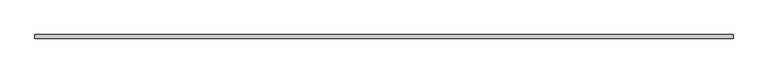
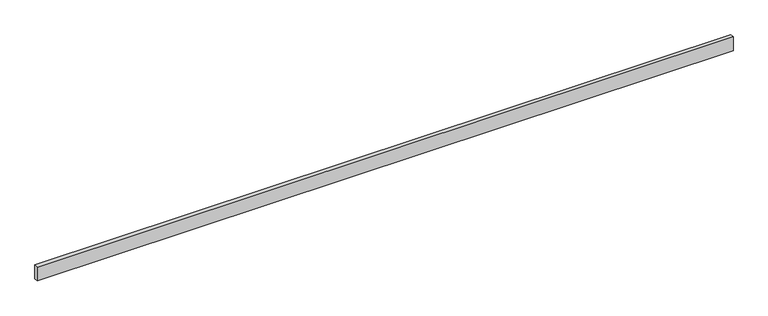
"""IFC4 building model written with IfcOpenShell, lengths in millimetres: proxy geometry, Generic Models 7:Generic Models 1:337419:Generic Models 1:337419 : Generic Models 7:Generic Models 1:337419:19 : Generic Models 7:Generic Models 1:337419:Generic Models 1:337419 : Generic Models 7:Generic Models 1:337419:301336."""

import ifcopenshell
import ifcopenshell.guid

model = None  # the IFC model being written
_history = None  # IfcOwnerHistory: only IFC2X3 demands one
_inside = {}  # id of a spatial element -> (the spatial element, [elements in it])
_under = {}  # id of a project, library or spatial element -> (it, [spatial elements below it])
_declared = {}  # id of a project -> (the project, [libraries it declares])
_typed = {}  # id of a type object -> (the type object, [elements of that type])
_made_of = {}  # id of a material, layer set ... -> (it, [elements and type objects made of it])


def new_model(schema):
    """Start an empty IFC model of exactly this schema.

    Asked for "IFC4X3", IfcOpenShell would pick the latest addendum, in which some entities
    have other attributes; the version numbers below select the first issue.
    IFC2X3 requires an IfcOwnerHistory on every rooted entity: one is made here for all.
    """
    global model, _history
    if schema == "IFC4X3":
        model = ifcopenshell.file(schema_version=(4, 3, 0, 0))
    else:
        model = ifcopenshell.file(schema=schema)
    _inside.clear()
    _under.clear()
    _declared.clear()
    _typed.clear()
    _made_of.clear()
    _history = None
    if model.schema == "IFC2X3":
        org = make("IfcOrganization", Name="unknown")
        user = make(
            "IfcPersonAndOrganization",
            ThePerson=make("IfcPerson", FamilyName="unknown"),
            TheOrganization=org,
        )
        app = make(
            "IfcApplication",
            ApplicationDeveloper=org,
            Version="unknown",
            ApplicationFullName="unknown",
            ApplicationIdentifier="unknown",
        )
        _history = make(
            "IfcOwnerHistory",
            OwningUser=user,
            OwningApplication=app,
            ChangeAction="ADDED",
            CreationDate=0,
        )
    return model


def make(cls, **values):
    """One entity of the class cls with the attributes given. An attribute that is None is left unset."""
    return model.create_entity(
        cls, **{name: value for name, value in values.items() if value is not None}
    )


def rooted(cls, **values):
    """An entity with a GlobalId (a new one), such as an element, a storey or a relation."""
    return make(cls, GlobalId=ifcopenshell.guid.new(), OwnerHistory=_history, **values)


def si_unit(unit_type, name, prefix=None):
    """IfcSIUnit, for example si_unit("LENGTHUNIT", "METRE", prefix="MILLI")."""
    return make("IfcSIUnit", UnitType=unit_type, Prefix=prefix, Name=name)


def assignment(units):
    """IfcUnitAssignment: the units of a project."""
    return None if units is None else make("IfcUnitAssignment", Units=units)


def point(xyz):
    """IfcCartesianPoint."""
    return None if xyz is None else make("IfcCartesianPoint", Coordinates=xyz)


def direction(xyz):
    """IfcDirection."""
    return None if xyz is None else make("IfcDirection", DirectionRatios=xyz)


def frame(location, z_axis=None, x_axis=None):
    """IfcAxis2Placement3D, a coordinate frame: its origin and axes. An axis left out is left unset."""
    return make(
        "IfcAxis2Placement3D",
        Location=point(location),
        Axis=direction(z_axis),
        RefDirection=direction(x_axis),
    )


def origin():
    """The frame at (0, 0, 0) with its axes left unset."""
    return frame((0.0, 0.0, 0.0))


def place(relative_to, where):
    """IfcLocalPlacement: puts the frame where relative to a parent placement (None: the world)."""
    return make(
        "IfcLocalPlacement", PlacementRelTo=relative_to, RelativePlacement=where
    )


def context(
    kind, dimensions, precision=None, world=None, true_north=None, identifier=None
):
    """IfcGeometricRepresentationContext, for example the 3D "Model" context."""
    return make(
        "IfcGeometricRepresentationContext",
        ContextIdentifier=identifier,
        ContextType=kind,
        CoordinateSpaceDimension=dimensions,
        Precision=precision,
        WorldCoordinateSystem=world,
        TrueNorth=true_north,
    )


def project(units=None, contexts=None):
    """IfcProject with its units and contexts."""
    return rooted(
        "IfcProject",
        Name="project",
        RepresentationContexts=contexts,
        UnitsInContext=assignment(units),
    )


def spatial(cls, under=None, at=None, **own):
    """A site, building, storey or space (cls), placed at a placement, below another one or the project."""
    s = rooted(cls, ObjectPlacement=at, **own)
    if under is not None:
        _under.setdefault(under.id(), (under, []))[1].append(s)
    return s


def polyline(points):
    """IfcPolyline through the points."""
    return make("IfcPolyline", Points=[point(p) for p in points])


def outline(outer, holes=None, kind="AREA"):
    """IfcArbitraryClosedProfileDef: a profile drawn as a closed curve; with holes, ...WithVoids."""
    if holes is None:
        return make("IfcArbitraryClosedProfileDef", ProfileType=kind, OuterCurve=outer)
    return make(
        "IfcArbitraryProfileDefWithVoids",
        ProfileType=kind,
        OuterCurve=outer,
        InnerCurves=holes,
    )


def extrude(swept, where, along, depth):
    """IfcExtrudedAreaSolid: the profile swept, set in the frame where, extruded along a direction by depth."""
    return make(
        "IfcExtrudedAreaSolid",
        SweptArea=swept,
        Position=where,
        ExtrudedDirection=direction(along),
        Depth=depth,
    )


def shape(context_of_items, identifier, shape_type, items):
    """IfcShapeRepresentation: the items that make up one representation, for example the "Body"."""
    return make(
        "IfcShapeRepresentation",
        ContextOfItems=context_of_items,
        RepresentationIdentifier=identifier,
        RepresentationType=shape_type,
        Items=items,
    )


def source(mapping_origin, context_of_items, identifier, shape_type, items):
    """IfcRepresentationMap: a shape defined once, which mapped items show again and again."""
    return make(
        "IfcRepresentationMap",
        MappingOrigin=mapping_origin,
        MappedRepresentation=shape(context_of_items, identifier, shape_type, items),
    )


def transform(
    local_origin,
    x_axis=None,
    y_axis=None,
    z_axis=None,
    scale=None,
    scale2=None,
    scale3=None,
    uniform=True,
):
    """IfcCartesianTransformationOperator3D, or its non-uniform kind. x_axis, y_axis, z_axis: its Axis1, 2, 3."""
    if uniform:
        return make(
            "IfcCartesianTransformationOperator3D",
            Axis1=direction(x_axis),
            Axis2=direction(y_axis),
            LocalOrigin=point(local_origin),
            Scale=scale,
            Axis3=direction(z_axis),
        )
    return make(
        "IfcCartesianTransformationOperator3DnonUniform",
        Axis1=direction(x_axis),
        Axis2=direction(y_axis),
        LocalOrigin=point(local_origin),
        Scale=scale,
        Axis3=direction(z_axis),
        Scale2=scale2,
        Scale3=scale3,
    )


def mapped(mapping_source, mapping_target):
    """IfcMappedItem: shows the shape of a source again, moved by a transform."""
    return make(
        "IfcMappedItem", MappingSource=mapping_source, MappingTarget=mapping_target
    )


def made_of(thing, what):
    """Note that an element or type object is made of a material, layer set ...; save() writes the relation."""
    if what is not None:
        _made_of.setdefault(what.id(), (what, []))[1].append(thing)
    return thing


def element(
    cls,
    number,
    at=None,
    inside=None,
    cuts=None,
    type_object=None,
    material=None,
    context=None,
    identifier="Body",
    shape_type=None,
    held_by="IfcProductDefinitionShape",
    body=None,
    shapes=None,
    **own,
):
    """One element of the class cls, such as IfcWall. Its Tag is "e" and its number.

    at: its placement. inside: the storey or other place that contains it. cuts: it is an
    opening in that element (IfcRelVoidsElement). A single representation is given by context,
    identifier, shape_type and body (its items); several are given by shapes. held_by: the class
    of the entity that holds the representations. save() writes the other relations.
    """
    e = rooted(cls, Tag="e%d" % number, ObjectPlacement=at, **own)
    if body is not None:
        shapes = [shape(context, identifier, shape_type, body)]
    if shapes is not None:
        e.Representation = make(held_by, Representations=shapes)
    if inside is not None:
        _inside.setdefault(inside.id(), (inside, []))[1].append(e)
    if cuts is not None:
        rooted(
            "IfcRelVoidsElement", RelatingBuildingElement=cuts, RelatedOpeningElement=e
        )
    if type_object is not None:
        _typed.setdefault(type_object.id(), (type_object, []))[1].append(e)
    return made_of(e, material)


def aggregate(whole, parts):
    """IfcRelAggregates: a whole, such as a stair, and the parts it consists of."""
    return rooted("IfcRelAggregates", RelatingObject=whole, RelatedObjects=parts)


def save(model, path):
    """Write the relations noted so far, then the file.

    IfcRelAggregates (storeys below a building ...), IfcRelContainedInSpatialStructure (elements
    in a storey), IfcRelDefinesByType, IfcRelAssociatesMaterial and IfcRelDeclares: one each for
    every whole, place, type object, material and project.
    """
    for whole, parts in _under.values():
        aggregate(whole, parts)
    for where, things in _inside.values():
        rooted(
            "IfcRelContainedInSpatialStructure",
            RelatedElements=things,
            RelatingStructure=where,
        )
    for kind, things in _typed.values():
        rooted("IfcRelDefinesByType", RelatedObjects=things, RelatingType=kind)
    for what, things in _made_of.values():
        rooted("IfcRelAssociatesMaterial", RelatedObjects=things, RelatingMaterial=what)
    for by, libraries in _declared.values():
        rooted("IfcRelDeclares", RelatingContext=by, RelatedDefinitions=libraries)
    model.write(path)


def generic_models_e323b401(model_context):
    return source(origin(), model_context, "Body", "SweptSolid", [
        extrude(outline(polyline([(596182.8367242, -536531.8913358), (596182.8367242, -536557.2913358), (591306.0367242, -536557.2913358), (591306.0367242, -536531.8913358), (596182.8367242, -536531.8913358)])), frame((0.0, 0.0, 6056.1140625), z_axis=(0.0, 0.0, 1.0), x_axis=(1.0, 0.0, 0.0)), (0.0, 0.0, 1.0), 101.6),
    ])


if __name__ == "__main__":
    model = new_model("IFC4")
    model_context = context("Model", 3, world=origin())
    ifc_project = project(units=[si_unit("LENGTHUNIT", "METRE", prefix="MILLI")], contexts=[model_context])
    site = spatial("IfcSite", under=ifc_project)
    building = spatial("IfcBuilding", under=site)
    placement = place(None, origin())
    generic_models_shape = generic_models_e323b401(model_context)
    element("IfcBuildingElementProxy", 1, Name="Generic Models 7:Generic Models 1:337419:Generic Models 1:337419 : Generic Models 7:Generic Models 1:337419:19 : Generic Models 7:Generic Models 1:337419:Generic Models 1:337419 : Generic Models 7:Generic Models 1:337419:301336", ObjectType="Generic Models 7:Generic Models 1:337419:Generic Models 1:337419 : Generic Models 7:Generic Models 1:337419:19 : Generic Models 7:Generic Models 1:337419:Generic Models 1:337419 : Generic Models 7:Generic Models 1:337419:301336", at=placement, inside=building, context=model_context, shape_type="MappedRepresentation", body=[
        mapped(generic_models_shape, transform((0.0, 0.0, 0.0), x_axis=(1.0, 0.0, 0.0), y_axis=(0.0, 1.0, 0.0), z_axis=(0.0, 0.0, 1.0))),
    ])
    save(model, "model.ifc")

# Revit data of these elements
# Type "Generic Models 7:Generic Models 1:337419:Generic Models 1:337419 : Generic Models 7:Generic Models 1:337419:19 : Generic Models 7:Generic Models 1:337419:Generic Models 1:337419 : Generic Models 7:Generic Models 1:337419:301336"
#   NameOverride = "Generic Models 7:Generic Models 1:337419:Generic Models 1:337419 : Generic Models 7:Generic Models 1:337419:301336"
#   ObjectTypeOverride = "Generic Models 1:337419 : Generic Models 7:Generic Models 1:337419"
#   Reference = "Generic Models 1"
#   Tag = "301336"
# Element 1 (IfcBuildingElementProxy, "Generic Models 7:Generic Models 1:337419:Generic Models 1:337419 : Generic Models 7:Generic Models 1:337419:19 : Generic Models 7:Generic Models 1:337419:Generic Models 1:337419 : Generic Models 7:Generic Models 1:337419:301336")
#   Materials on its faces: "1\" THERMAL SPACER @ GIRT"
# Materials
#   "1\" THERMAL SPACER @ GIRT": class "Unassigned", colour RGB 205 188 106, transparency 0, Cost = 0
